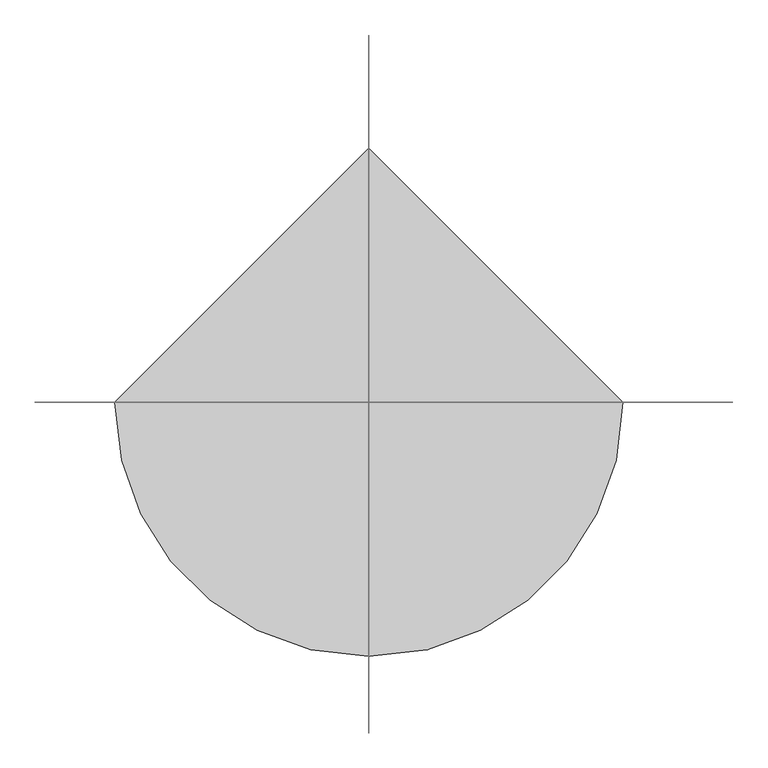
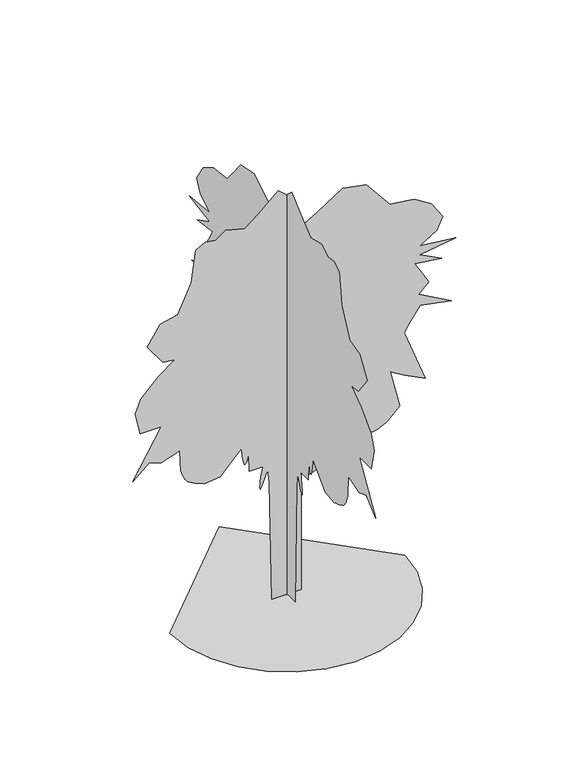
"""IFC4 building model written with IfcOpenShell, lengths in millimetres: proxy geometry, windmill palm 26123 : windmill palm 26123."""

import ifcopenshell
import ifcopenshell.guid

model = None  # the IFC model being written
_history = None  # IfcOwnerHistory: only IFC2X3 demands one
_inside = {}  # id of a spatial element -> (the spatial element, [elements in it])
_under = {}  # id of a project, library or spatial element -> (it, [spatial elements below it])
_declared = {}  # id of a project -> (the project, [libraries it declares])
_typed = {}  # id of a type object -> (the type object, [elements of that type])
_made_of = {}  # id of a material, layer set ... -> (it, [elements and type objects made of it])


def new_model(schema):
    """Start an empty IFC model of exactly this schema.

    Asked for "IFC4X3", IfcOpenShell would pick the latest addendum, in which some entities
    have other attributes; the version numbers below select the first issue.
    IFC2X3 requires an IfcOwnerHistory on every rooted entity: one is made here for all.
    """
    global model, _history
    if schema == "IFC4X3":
        model = ifcopenshell.file(schema_version=(4, 3, 0, 0))
    else:
        model = ifcopenshell.file(schema=schema)
    _inside.clear()
    _under.clear()
    _declared.clear()
    _typed.clear()
    _made_of.clear()
    _history = None
    if model.schema == "IFC2X3":
        org = make("IfcOrganization", Name="unknown")
        user = make(
            "IfcPersonAndOrganization",
            ThePerson=make("IfcPerson", FamilyName="unknown"),
            TheOrganization=org,
        )
        app = make(
            "IfcApplication",
            ApplicationDeveloper=org,
            Version="unknown",
            ApplicationFullName="unknown",
            ApplicationIdentifier="unknown",
        )
        _history = make(
            "IfcOwnerHistory",
            OwningUser=user,
            OwningApplication=app,
            ChangeAction="ADDED",
            CreationDate=0,
        )
    return model


def make(cls, **values):
    """One entity of the class cls with the attributes given. An attribute that is None is left unset."""
    return model.create_entity(
        cls, **{name: value for name, value in values.items() if value is not None}
    )


def rooted(cls, **values):
    """An entity with a GlobalId (a new one), such as an element, a storey or a relation."""
    return make(cls, GlobalId=ifcopenshell.guid.new(), OwnerHistory=_history, **values)


def si_unit(unit_type, name, prefix=None):
    """IfcSIUnit, for example si_unit("LENGTHUNIT", "METRE", prefix="MILLI")."""
    return make("IfcSIUnit", UnitType=unit_type, Prefix=prefix, Name=name)


def assignment(units):
    """IfcUnitAssignment: the units of a project."""
    return None if units is None else make("IfcUnitAssignment", Units=units)


def point(xyz):
    """IfcCartesianPoint."""
    return None if xyz is None else make("IfcCartesianPoint", Coordinates=xyz)


def direction(xyz):
    """IfcDirection."""
    return None if xyz is None else make("IfcDirection", DirectionRatios=xyz)


def frame(location, z_axis=None, x_axis=None):
    """IfcAxis2Placement3D, a coordinate frame: its origin and axes. An axis left out is left unset."""
    return make(
        "IfcAxis2Placement3D",
        Location=point(location),
        Axis=direction(z_axis),
        RefDirection=direction(x_axis),
    )


def origin():
    """The frame at (0, 0, 0) with its axes left unset."""
    return frame((0.0, 0.0, 0.0))


def place(relative_to, where):
    """IfcLocalPlacement: puts the frame where relative to a parent placement (None: the world)."""
    return make(
        "IfcLocalPlacement", PlacementRelTo=relative_to, RelativePlacement=where
    )


def context(
    kind, dimensions, precision=None, world=None, true_north=None, identifier=None
):
    """IfcGeometricRepresentationContext, for example the 3D "Model" context."""
    return make(
        "IfcGeometricRepresentationContext",
        ContextIdentifier=identifier,
        ContextType=kind,
        CoordinateSpaceDimension=dimensions,
        Precision=precision,
        WorldCoordinateSystem=world,
        TrueNorth=true_north,
    )


def project(units=None, contexts=None):
    """IfcProject with its units and contexts."""
    return rooted(
        "IfcProject",
        Name="project",
        RepresentationContexts=contexts,
        UnitsInContext=assignment(units),
    )


def spatial(cls, under=None, at=None, **own):
    """A site, building, storey or space (cls), placed at a placement, below another one or the project."""
    s = rooted(cls, ObjectPlacement=at, **own)
    if under is not None:
        _under.setdefault(under.id(), (under, []))[1].append(s)
    return s


def point_list(points):
    """IfcCartesianPointList2D or 3D."""
    cls = (
        "IfcCartesianPointList2D" if len(points[0]) == 2 else "IfcCartesianPointList3D"
    )
    return make(cls, CoordList=points)


def triangles(points, corners, closed=None, point_numbers=None):
    """IfcTriangulatedFaceSet: each triangle names its three corners, points numbered from 1."""
    return make(
        "IfcTriangulatedFaceSet",
        Coordinates=point_list(points),
        Closed=closed,
        CoordIndex=corners,
        PnIndex=point_numbers,
    )


def shape(context_of_items, identifier, shape_type, items):
    """IfcShapeRepresentation: the items that make up one representation, for example the "Body"."""
    return make(
        "IfcShapeRepresentation",
        ContextOfItems=context_of_items,
        RepresentationIdentifier=identifier,
        RepresentationType=shape_type,
        Items=items,
    )


def source(mapping_origin, context_of_items, identifier, shape_type, items):
    """IfcRepresentationMap: a shape defined once, which mapped items show again and again."""
    return make(
        "IfcRepresentationMap",
        MappingOrigin=mapping_origin,
        MappedRepresentation=shape(context_of_items, identifier, shape_type, items),
    )


def transform(
    local_origin,
    x_axis=None,
    y_axis=None,
    z_axis=None,
    scale=None,
    scale2=None,
    scale3=None,
    uniform=True,
):
    """IfcCartesianTransformationOperator3D, or its non-uniform kind. x_axis, y_axis, z_axis: its Axis1, 2, 3."""
    if uniform:
        return make(
            "IfcCartesianTransformationOperator3D",
            Axis1=direction(x_axis),
            Axis2=direction(y_axis),
            LocalOrigin=point(local_origin),
            Scale=scale,
            Axis3=direction(z_axis),
        )
    return make(
        "IfcCartesianTransformationOperator3DnonUniform",
        Axis1=direction(x_axis),
        Axis2=direction(y_axis),
        LocalOrigin=point(local_origin),
        Scale=scale,
        Axis3=direction(z_axis),
        Scale2=scale2,
        Scale3=scale3,
    )


def mapped(mapping_source, mapping_target):
    """IfcMappedItem: shows the shape of a source again, moved by a transform."""
    return make(
        "IfcMappedItem", MappingSource=mapping_source, MappingTarget=mapping_target
    )


def made_of(thing, what):
    """Note that an element or type object is made of a material, layer set ...; save() writes the relation."""
    if what is not None:
        _made_of.setdefault(what.id(), (what, []))[1].append(thing)
    return thing


def element(
    cls,
    number,
    at=None,
    inside=None,
    cuts=None,
    type_object=None,
    material=None,
    context=None,
    identifier="Body",
    shape_type=None,
    held_by="IfcProductDefinitionShape",
    body=None,
    shapes=None,
    **own,
):
    """One element of the class cls, such as IfcWall. Its Tag is "e" and its number.

    at: its placement. inside: the storey or other place that contains it. cuts: it is an
    opening in that element (IfcRelVoidsElement). A single representation is given by context,
    identifier, shape_type and body (its items); several are given by shapes. held_by: the class
    of the entity that holds the representations. save() writes the other relations.
    """
    e = rooted(cls, Tag="e%d" % number, ObjectPlacement=at, **own)
    if body is not None:
        shapes = [shape(context, identifier, shape_type, body)]
    if shapes is not None:
        e.Representation = make(held_by, Representations=shapes)
    if inside is not None:
        _inside.setdefault(inside.id(), (inside, []))[1].append(e)
    if cuts is not None:
        rooted(
            "IfcRelVoidsElement", RelatingBuildingElement=cuts, RelatedOpeningElement=e
        )
    if type_object is not None:
        _typed.setdefault(type_object.id(), (type_object, []))[1].append(e)
    return made_of(e, material)


def aggregate(whole, parts):
    """IfcRelAggregates: a whole, such as a stair, and the parts it consists of."""
    return rooted("IfcRelAggregates", RelatingObject=whole, RelatedObjects=parts)


def save(model, path):
    """Write the relations noted so far, then the file.

    IfcRelAggregates (storeys below a building ...), IfcRelContainedInSpatialStructure (elements
    in a storey), IfcRelDefinesByType, IfcRelAssociatesMaterial and IfcRelDeclares: one each for
    every whole, place, type object, material and project.
    """
    for whole, parts in _under.values():
        aggregate(whole, parts)
    for where, things in _inside.values():
        rooted(
            "IfcRelContainedInSpatialStructure",
            RelatedElements=things,
            RelatingStructure=where,
        )
    for kind, things in _typed.values():
        rooted("IfcRelDefinesByType", RelatedObjects=things, RelatingType=kind)
    for what, things in _made_of.values():
        rooted("IfcRelAssociatesMaterial", RelatedObjects=things, RelatingMaterial=what)
    for by, libraries in _declared.values():
        rooted("IfcRelDeclares", RelatingContext=by, RelatedDefinitions=libraries)
    model.write(path)


def entourage_d7a905c7(model_context):
    return source(origin(), model_context, "Body", "Tessellation", [
        triangles([(-0.2241189, -80.6803134, 0.0560704), (-0.2241181, -93.4507094, 708.3955685), (-0.2241176, -102.9729479, 784.5729681), (-0.2241171, -112.4304103, 759.6428038), (-0.2241163, -121.4992608, 736.1299221), (-0.2241158, -129.7908604, 715.4466642), (-0.2241156, -136.916343, 699.0127836), (-0.2241151, -142.4870876, 688.2406214), (-0.2241151, -146.1147278, 684.5474602), (-0.2241148, -147.4101338, 689.3505827), (-0.2241148, -146.9475984, 700.5392893), (-0.2241151, -145.6519381, 714.7252693), (-0.2241151, -143.662352, 731.4105881), (-0.2241153, -141.1175219, 750.0923693), (-0.2241156, -138.1563745, 770.2752216), (-0.2241156, -134.9173553, 791.458885), (-0.2241158, -131.5396545, 813.1404104), (-0.2241113, -207.7180624, 813.1404104), (-0.224111, -210.8920511, 914.7103008), (-0.2241108, -214.9636775, 900.580204), (-0.2241105, -218.9799477, 887.367057), (-0.2241105, -222.88496, 875.9827955), (-0.2241103, -226.6235945, 867.3493109), (-0.22411, -230.1402221, 862.3810095), (-0.2241097, -233.3789961, 861.9923704), (-0.2241095, -236.2847599, 867.1003435), (-0.2241095, -238.9129061, 876.4653969), (-0.2241092, -241.3744383, 887.9944897), (-0.2241092, -243.6972616, 901.3295042), (-0.224109, -245.9088635, 916.1097794), (-0.224109, -248.0373855, 931.9696398), (-0.2241087, -250.1102786, 948.5533659), (-0.2241087, -252.1552483, 965.4977531), (-0.2241016, -372.7715778, 838.5329012), (-0.2240963, -461.6464946, 829.010372), (-0.224095, -479.2563572, 835.8125004), (-0.224094, -496.4217339, 842.6147015), (-0.2240932, -512.6981023, 849.4168299), (-0.2240922, -527.64352, 856.2164148), (-0.2240914, -540.8134646, 863.0185432), (-0.2240907, -551.7608706, 869.8206717), (-0.2240902, -560.0413244, 876.6228727), (-0.2240899, -566.4726179, 884.1641275), (-0.2240897, -572.238436, 893.0389492), (-0.2240892, -577.4480018, 903.0236595), (-0.2240889, -582.2155887, 913.8974871), (-0.2240887, -586.6479126, 925.4367537), (-0.2240884, -590.8567037, 937.4204699), (-0.2240881, -594.9562717, 949.6252481), (-0.2240879, -601.3062839, 1073.4150759), (-0.2240815, -706.0511621, 1038.5001286), (-0.2240775, -775.8810568, 1063.8925467), (-0.2240719, -867.928418, 981.3677147), (-0.2240815, -706.0511621, 1254.3398609), (-0.2240744, -826.6659657, 1254.3398609), (-0.2240727, -855.233408, 1381.3021694), (-0.2240747, -823.4909414, 1460.6545933), (-0.2240805, -725.0961479, 1562.224411), (-0.2240861, -629.8712191, 1632.0567764), (-0.2240821, -699.7011137, 1641.5768349), (-0.224077, -785.4035133, 1759.0190849), (-0.2240813, -712.3985945, 1873.2865288), (-0.2240871, -614.0012575, 1895.5039227), (-0.2240917, -537.8238579, 2060.5586735), (-0.2240932, -512.4314034, 2247.8284927), (-0.2240963, -458.4714704, 2276.3959351), (-0.2240998, -398.1640686, 2266.8734058), (-0.2241034, -341.0291113, 2308.1358582), (-0.2241097, -233.1107712, 2279.5708866), (-0.2241143, -156.9326267, 2339.8783974), (-0.2241212, -42.6652782, 2438.2757343), (-0.2241265, 46.2093524, 2358.9233105), (-0.2241265, 46.2093524, 2263.6984543), (-0.2241298, 103.3427746, 2190.6960789), (-0.2241346, 182.6954255, 2235.1334827), (-0.224143, 322.3549604, 2327.1809166), (-0.2241509, 455.6672811, 2301.7884258), (-0.2241557, 538.1921494, 2200.2186081), (-0.2241588, 588.979638, 2136.7361458), (-0.2241672, 728.6394636, 2117.6910873), (-0.224173, 827.0368006, 2057.3837219), (-0.2241768, 890.5167194, 1958.986385), (-0.2241748, 855.6017721, 1889.1564903), (-0.2241689, 760.3793867, 1828.8489796), (-0.2241811, 963.5216383, 1806.6315857), (-0.2241689, 760.3793867, 1774.8890465), (-0.2241763, 884.1692144, 1711.4067295), (-0.2241674, 731.8118717, 1730.4516426), (-0.224172, 811.1642956, 1593.9668049), (-0.2241687, 754.0318817, 1540.0068718), (-0.2241796, 938.1291475, 1435.2621025), (-0.2241692, 763.5544109, 1470.1769772), (-0.2241654, 700.0719486, 1384.477121), (-0.2241636, 671.5045063, 1336.8647655), (-0.224171, 792.1193098, 1022.630167), (-0.2241639, 674.6795305, 1079.7650517), (-0.224159, 592.1520824, 1130.5500332), (-0.2241621, 646.1120155, 908.3627958), (-0.2241583, 579.4571451, 841.7079254), (-0.2241575, 566.5462689, 834.2758209), (-0.2241567, 553.721761, 827.1511105), (-0.224156, 541.0623593, 820.6359558), (-0.2241552, 528.6518887, 815.0378237), (-0.2241544, 516.5766809, 810.6613466), (-0.2241537, 504.9155105, 807.8089771), (-0.2241532, 493.7572526, 806.7929054), (-0.2241524, 482.6879065, 807.6260668), (-0.2241519, 471.2883479, 809.9577559), (-0.2241511, 459.6093733, 813.5392233), (-0.2241504, 447.7094456, 818.1188129), (-0.2241496, 435.6418682, 823.4503189), (-0.2241489, 423.4625244, 829.2796143), (-0.2241481, 411.2298409, 835.357877), (-0.2241481, 407.7779803, 839.4116993), (-0.2241478, 404.0213056, 843.2979446), (-0.2241476, 399.6524952, 846.8514341), (-0.2241471, 394.3692784, 849.9070616), (-0.2241468, 387.8643339, 852.2946339), (-0.2241463, 379.8302676, 853.8491175), (-0.2241458, 369.9674249, 854.4028627), (-0.224145, 357.1403735, 855.883659), (-0.224144, 340.8157522, 860.0289728), (-0.2241428, 321.5777186, 866.3967527), (-0.2241415, 300.0079778, 874.5400057), (-0.2241402, 276.6881621, 884.0168255), (-0.2241387, 252.2014664, 894.3800737), (-0.2241372, 227.1326114, 905.1877716), (-0.2241349, 185.8694142, 857.577887), (-0.2241349, 185.8694142, 778.2254631), (-0.2241362, 208.0876256, 702.0480635), (-0.2241316, 131.9097354, 676.6556454), (-0.2241288, 87.4725496, 800.4429296), (-0.2241293, 88.096376, 0.0), (-666.8181644, -2.5e-06, 0.2128606), (-649.2007078, -152.6793797, 0.2128611), (-599.0329851, -292.8908795, 0.2128626), (-520.3257617, -416.61723, 0.2128649), (-417.1023385, -519.8431603, 0.2128679), (-293.3760243, -598.5478403, 0.2128717), (-153.1642702, -648.715563, 0.2128758), (-0.4850755, -666.3330196, 0.2128804), (152.1942349, -648.715563, 0.2128849), (292.4057347, -598.5478403, 0.212889), (416.1320852, -519.8406169, 0.2128928), (519.3580155, -416.61723, 0.2128959), (598.0626955, -292.8908795, 0.2128981), (648.2304182, -152.6791254, 0.2128997), (665.8478748, 5.82e-05, 0.2129002), (-0.4851924, 666.3330196, 0.2128804), (-89.341994, 0.0001455, 0.1894216), (-102.11239, 0.0001057, 708.5276825), (-111.6346285, 9.96e-05, 784.7075529), (-121.0920909, 0.0001025, 759.7773886), (-130.1609414, 0.0001023, 736.2619635), (-138.4522867, 0.0001051, 715.581249), (-145.5777693, 0.000105, 699.144825), (-151.1487682, 0.0001048, 688.3726627), (-154.7761631, 0.0001075, 684.682045), (-156.0718144, 0.0001043, 689.4852402), (-155.6090338, 0.0001041, 700.6714033), (-154.3136187, 0.0001037, 714.8573833), (-152.3240326, 0.0001034, 731.5426294), (-149.7792025, 0.0001031, 750.2269541), (-146.8178008, 9.98e-05, 770.4098791), (-143.5790359, 9.95e-05, 791.590999), (-140.2013351, 9.92e-05, 813.2725245), (-216.3794887, 9.82e-05, 813.2725245), (-219.5534773, 9.2e-05, 914.8448856), (-223.6253582, 9.2e-05, 900.7147888), (-227.6413739, 9.5e-05, 887.4991711), (-231.5466406, 9.5e-05, 876.1173803), (-235.2852751, 9.49e-05, 867.4838957), (-238.8016665, 9.47e-05, 862.5131235), (-242.0406767, 9.44e-05, 862.1244844), (-244.9461861, 9.4e-05, 867.2324575), (-247.5745867, 9.35e-05, 876.5974382), (-250.0361189, 9.29e-05, 888.1290745), (-252.358706, 9.23e-05, 901.464089), (-254.5697811, 9.17e-05, 916.2418934), (-256.6983031, 9.1e-05, 932.1042246), (-258.7709418, 9.04e-05, 948.6854073), (-260.8156571, 8.97e-05, 965.6297945), (-381.4330041, 9.73e-05, 838.667486), (-470.3079208, 9.84e-05, 829.1450294), (-487.9177835, 9.66e-05, 835.9446144), (-505.0831601, 9.78e-05, 842.7467428), (-521.3595285, 9.61e-05, 849.5488712), (-536.3049462, 9.46e-05, 856.3510723), (-549.4748909, 9.61e-05, 863.1532007), (-560.4222968, 9.49e-05, 869.9527857), (-568.7027507, 9.4e-05, 876.7549141), (-575.1340442, 9.32e-05, 884.2962416), (-580.8998623, 9.24e-05, 893.1709906), (-586.109428, 9.17e-05, 903.1557735), (-590.8770149, 9.38e-05, 914.0295284), (-595.3093389, 9.31e-05, 925.568795), (-599.5181299, 9.23e-05, 937.5525839), (-603.617698, 9.16e-05, 949.759833), (-609.9677101, 8.15e-05, 1073.5496607), (-714.7125521, 8.49e-05, 1038.6347134), (-784.5424467, 8.37e-05, 1064.0272041), (-876.5898079, 8.96e-05, 981.4997561), (-714.7125521, 7.26e-05, 1254.4719749), (-835.3274282, 7.35e-05, 1254.4719749), (-863.8948706, 6.42e-05, 1381.4367542), (-832.152404, 5.89e-05, 1460.7891781), (-733.7575378, 5.3e-05, 1562.3589958), (-638.532609, 5.06e-05, 1632.1888905), (-708.3625763, 4.99e-05, 1641.7114197), (-794.0649759, 4.17e-05, 1759.1538151), (-721.0600571, 3.61e-05, 1873.4184975), (-622.6626474, 3.25e-05, 1895.6385075), (-546.4852841, 2.27e-05, 2060.6907875), (-521.0928297, 1.36e-05, 2247.9630775), (-467.1328966, 1.17e-05, 2276.5305199), (-406.8254949, 1.15e-05, 2267.0079906), (-349.6905375, 9.6e-06, 2308.270443), (-241.7724518, 1.13e-05, 2279.7030006), (-165.5940529, 7.6e-06, 2340.0103661), (-51.3267045, 3e-07, 2438.4078484), (37.5476695, 7.7e-06, 2359.0554245), (37.5476695, 1.34e-05, 2263.8330391), (94.6810849, 1.78e-05, 2190.8281929), (174.0337449, 1.48e-05, 2235.2655968), (313.6935342, 7e-06, 2327.3155014), (447.0058548, 1.09e-05, 2301.9230106), (529.5307231, 1.55e-05, 2200.3505768), (580.3182117, 1.9e-05, 2136.8682598), (719.978001, 2.04e-05, 2117.8258175), (818.3728672, 2.51e-05, 2057.515836), (881.8552568, 3.08e-05, 1959.1209698), (846.9403095, 3.56e-05, 1889.2910751), (751.7179241, 3.77e-05, 1828.9837097), (954.8601757, 3.9e-05, 1806.7636997), (751.7179241, 4.22e-05, 1775.0237766), (875.5077518, 4.35e-05, 1711.5413143), (723.1504818, 4.39e-05, 1730.5862274), (802.502833, 5.21e-05, 1594.0989189), (745.3704918, 5.45e-05, 1540.1416019), (929.4676849, 6.24e-05, 1435.3942165), (754.8929483, 6.03e-05, 1470.3117073), (691.4105587, 6.3e-05, 1384.609235), (662.8430437, 6.77e-05, 1336.9993504), (783.4579199, 8.5e-05, 1022.7647518), (666.0180679, 8.15e-05, 1079.8971657), (583.4906562, 7.85e-05, 1130.6820745), (637.4506256, 9.28e-05, 908.4973806), (570.7957189, 9.76e-05, 841.8399668), (557.8848427, 9.67e-05, 834.4104784), (545.0603348, 9.87e-05, 827.2831518), (532.4009331, 9.77e-05, 820.7706133), (519.9904624, 9.97e-05, 815.169865), (507.9152547, 9.88e-05, 810.7934607), (496.2540842, 9.78e-05, 807.9435619), (485.0932829, 9.98e-05, 806.9250195), (474.0264802, 9.87e-05, 807.7581808), (462.6269217, 9.77e-05, 810.0898699), (450.947947, 9.94e-05, 813.6712646), (439.0480193, 9.82e-05, 818.2534704), (426.980442, 9.7e-05, 823.5823603), (414.8010982, 9.86e-05, 829.4117283), (402.5684146, 9.74e-05, 835.4924618), (399.1165541, 9.69e-05, 839.5463568), (395.3598793, 9.65e-05, 843.4325294), (390.9910689, 9.6e-05, 846.9860189), (385.7078522, 9.54e-05, 850.0391029), (379.2029077, 9.48e-05, 852.4267479), (371.1688414, 9.69e-05, 853.9812315), (361.3059986, 9.6e-05, 854.5374475), (348.4789473, 9.48e-05, 856.0183165), (332.154326, 9.62e-05, 860.1635576), (312.9162924, 9.43e-05, 866.5288668), (291.3465516, 9.5e-05, 874.6721197), (268.0267359, 9.56e-05, 884.1488668), (243.5397858, 9.31e-05, 894.5146585), (218.4709308, 9.34e-05, 905.3224291), (177.2077336, 9.7e-05, 857.7099283), (177.2077336, 9.94e-05, 778.3575771), (199.4261993, 0.0001036, 702.1801775), (123.2483092, 0.0001063, 676.7876867), (78.8108599, 9.87e-05, 800.5775145), (79.4346863, 0.0001459, 0.1333563)], [[85, 84, 86], [53, 52, 54], [91, 90, 92], [87, 86, 88], [95, 94, 96], [96, 94, 97], [9, 8, 10], [52, 51, 54], [51, 50, 54], [1, 133, 2], [133, 132, 2], [2, 132, 3], [131, 130, 132], [130, 129, 132], [129, 128, 132], [18, 17, 19], [71, 70, 72], [72, 70, 73], [10, 8, 11], [8, 7, 11], [11, 7, 12], [7, 6, 12], [12, 6, 13], [6, 5, 13], [13, 5, 14], [5, 4, 14], [14, 4, 15], [4, 3, 15], [15, 3, 16], [16, 3, 17], [55, 54, 56], [89, 88, 90], [56, 54, 57], [57, 54, 58], [61, 60, 62], [62, 60, 63], [60, 59, 63], [25, 24, 26], [24, 23, 26], [26, 23, 27], [23, 22, 27], [27, 22, 28], [22, 21, 28], [28, 21, 29], [21, 20, 29], [29, 20, 30], [20, 19, 30], [30, 19, 31], [82, 81, 83], [83, 81, 84], [81, 80, 84], [80, 79, 84], [70, 69, 73], [98, 97, 99], [31, 19, 32], [99, 97, 100], [58, 54, 59], [100, 97, 101], [101, 97, 102], [102, 97, 103], [103, 97, 104], [104, 97, 105], [105, 97, 106], [106, 97, 107], [107, 97, 108], [108, 97, 109], [109, 97, 110], [110, 97, 111], [111, 97, 112], [112, 97, 113], [113, 97, 114], [114, 97, 115], [115, 97, 116], [116, 97, 117], [117, 97, 118], [118, 97, 119], [119, 97, 120], [120, 97, 121], [121, 97, 122], [122, 97, 123], [123, 97, 124], [124, 97, 125], [125, 97, 126], [126, 97, 127], [65, 64, 66], [66, 64, 67], [68, 67, 69], [67, 64, 69], [3, 132, 17], [73, 69, 74], [69, 64, 74], [64, 63, 74], [63, 59, 74], [17, 132, 19], [132, 128, 19], [128, 127, 19], [92, 90, 93], [76, 75, 77], [77, 75, 78], [78, 75, 79], [79, 75, 84], [75, 74, 84], [74, 59, 84], [84, 59, 86], [86, 59, 88], [88, 59, 90], [90, 59, 93], [93, 59, 94], [94, 59, 97], [97, 59, 127], [127, 59, 19], [32, 19, 33], [19, 59, 33], [59, 54, 33], [54, 50, 33], [33, 50, 34], [50, 49, 34], [34, 49, 35], [35, 49, 36], [36, 49, 37], [49, 48, 37], [37, 48, 38], [48, 47, 38], [38, 47, 39], [47, 46, 39], [39, 46, 40], [46, 45, 40], [45, 44, 40], [40, 44, 41], [44, 43, 41], [41, 43, 42], [148, 149, 134], [147, 148, 134], [147, 134, 135], [146, 147, 135], [146, 135, 136], [146, 136, 137], [145, 146, 137], [144, 145, 137], [144, 137, 138], [144, 138, 139], [144, 139, 140], [144, 140, 141], [144, 141, 142], [144, 142, 143], [233, 234, 235], [201, 202, 203], [239, 240, 241], [235, 236, 237], [243, 244, 245], [243, 245, 246], [157, 158, 159], [200, 201, 203], [199, 200, 203], [282, 150, 151], [281, 282, 151], [281, 151, 152], [279, 280, 281], [278, 279, 281], [277, 278, 281], [166, 167, 168], [219, 220, 221], [219, 221, 222], [157, 159, 160], [156, 157, 160], [156, 160, 161], [155, 156, 161], [155, 161, 162], [154, 155, 162], [154, 162, 163], [153, 154, 163], [153, 163, 164], [152, 153, 164], [152, 164, 165], [152, 165, 166], [203, 204, 205], [237, 238, 239], [203, 205, 206], [203, 206, 207], [209, 210, 211], [209, 211, 212], [208, 209, 212], [173, 174, 175], [172, 173, 175], [172, 175, 176], [171, 172, 176], [171, 176, 177], [170, 171, 177], [170, 177, 178], [169, 170, 178], [169, 178, 179], [168, 169, 179], [168, 179, 180], [230, 231, 232], [230, 232, 233], [229, 230, 233], [228, 229, 233], [218, 219, 222], [246, 247, 248], [168, 180, 181], [246, 248, 249], [203, 207, 208], [246, 249, 250], [246, 250, 251], [246, 251, 252], [246, 252, 253], [246, 253, 254], [246, 254, 255], [246, 255, 256], [246, 256, 257], [246, 257, 258], [246, 258, 259], [246, 259, 260], [246, 260, 261], [246, 261, 262], [246, 262, 263], [246, 263, 264], [246, 264, 265], [246, 265, 266], [246, 266, 267], [246, 267, 268], [246, 268, 269], [246, 269, 270], [246, 270, 271], [246, 271, 272], [246, 272, 273], [246, 273, 274], [246, 274, 275], [246, 275, 276], [213, 214, 215], [213, 215, 216], [216, 217, 218], [213, 216, 218], [281, 152, 166], [218, 222, 223], [213, 218, 223], [212, 213, 223], [208, 212, 223], [281, 166, 168], [277, 281, 168], [276, 277, 168], [239, 241, 242], [224, 225, 226], [224, 226, 227], [224, 227, 228], [224, 228, 233], [223, 224, 233], [208, 223, 233], [208, 233, 235], [208, 235, 237], [208, 237, 239], [208, 239, 242], [208, 242, 243], [208, 243, 246], [208, 246, 276], [208, 276, 168], [168, 181, 182], [208, 168, 182], [203, 208, 182], [199, 203, 182], [199, 182, 183], [198, 199, 183], [198, 183, 184], [198, 184, 185], [198, 185, 186], [197, 198, 186], [197, 186, 187], [196, 197, 187], [196, 187, 188], [195, 196, 188], [195, 188, 189], [194, 195, 189], [193, 194, 189], [193, 189, 190], [192, 193, 190], [192, 190, 191]], closed=False),
    ])


if __name__ == "__main__":
    model = new_model("IFC4")
    model_context = context("Model", 3, world=origin())
    ifc_project = project(units=[si_unit("LENGTHUNIT", "METRE", prefix="MILLI")], contexts=[model_context])
    site = spatial("IfcSite", under=ifc_project)
    building = spatial("IfcBuilding", under=site)
    placement = place(None, origin())
    entourage_shape = entourage_d7a905c7(model_context)
    element("IfcBuildingElementProxy", 1, Name="windmill palm 26123 : windmill palm 26123", ObjectType="windmill palm 26123 : windmill palm 26123", at=placement, inside=building, context=model_context, shape_type="MappedRepresentation", body=[
        mapped(entourage_shape, transform((0.0, 0.0, 0.0), x_axis=(1.0, 0.0, 0.0), y_axis=(0.0, 1.0, 0.0), z_axis=(0.0, 0.0, 1.0))),
    ])
    save(model, "model.ifc")

# Revit data of these elements
# Type "windmill palm 26123 : windmill palm 26123"
#   built-in parameter 1005195 = "RPC-16-G2MF-J1Q0-CAN1-N000-ST1L-LVER-AU"
#   Height = 0
